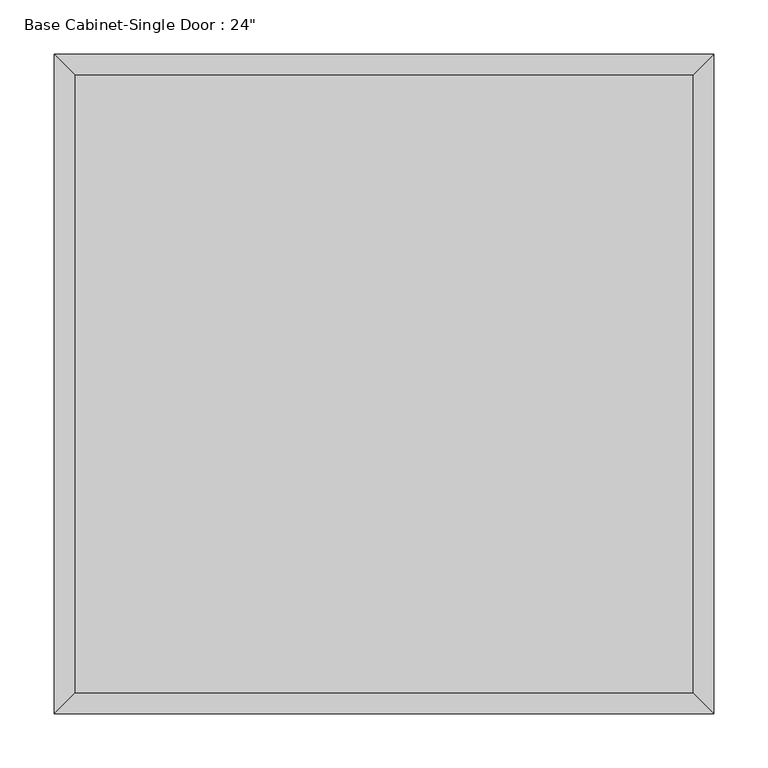
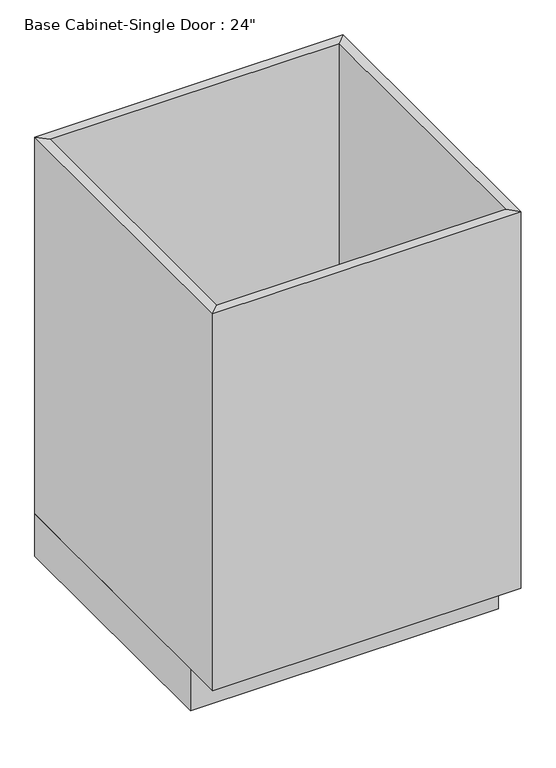
"""IFC4 building model written with IfcOpenShell, lengths in millimetres: furniture geometry."""

import ifcopenshell
import ifcopenshell.guid

model = None  # the IFC model being written
_history = None  # IfcOwnerHistory: only IFC2X3 demands one
_inside = {}  # id of a spatial element -> (the spatial element, [elements in it])
_under = {}  # id of a project, library or spatial element -> (it, [spatial elements below it])
_declared = {}  # id of a project -> (the project, [libraries it declares])
_typed = {}  # id of a type object -> (the type object, [elements of that type])
_made_of = {}  # id of a material, layer set ... -> (it, [elements and type objects made of it])


def new_model(schema):
    """Start an empty IFC model of exactly this schema.

    Asked for "IFC4X3", IfcOpenShell would pick the latest addendum, in which some entities
    have other attributes; the version numbers below select the first issue.
    IFC2X3 requires an IfcOwnerHistory on every rooted entity: one is made here for all.
    """
    global model, _history
    if schema == "IFC4X3":
        model = ifcopenshell.file(schema_version=(4, 3, 0, 0))
    else:
        model = ifcopenshell.file(schema=schema)
    _inside.clear()
    _under.clear()
    _declared.clear()
    _typed.clear()
    _made_of.clear()
    _history = None
    if model.schema == "IFC2X3":
        org = make("IfcOrganization", Name="unknown")
        user = make(
            "IfcPersonAndOrganization",
            ThePerson=make("IfcPerson", FamilyName="unknown"),
            TheOrganization=org,
        )
        app = make(
            "IfcApplication",
            ApplicationDeveloper=org,
            Version="unknown",
            ApplicationFullName="unknown",
            ApplicationIdentifier="unknown",
        )
        _history = make(
            "IfcOwnerHistory",
            OwningUser=user,
            OwningApplication=app,
            ChangeAction="ADDED",
            CreationDate=0,
        )
    return model


def make(cls, **values):
    """One entity of the class cls with the attributes given. An attribute that is None is left unset."""
    return model.create_entity(
        cls, **{name: value for name, value in values.items() if value is not None}
    )


def rooted(cls, **values):
    """An entity with a GlobalId (a new one), such as an element, a storey or a relation."""
    return make(cls, GlobalId=ifcopenshell.guid.new(), OwnerHistory=_history, **values)


def si_unit(unit_type, name, prefix=None):
    """IfcSIUnit, for example si_unit("LENGTHUNIT", "METRE", prefix="MILLI")."""
    return make("IfcSIUnit", UnitType=unit_type, Prefix=prefix, Name=name)


def assignment(units):
    """IfcUnitAssignment: the units of a project."""
    return None if units is None else make("IfcUnitAssignment", Units=units)


def point(xyz):
    """IfcCartesianPoint."""
    return None if xyz is None else make("IfcCartesianPoint", Coordinates=xyz)


def direction(xyz):
    """IfcDirection."""
    return None if xyz is None else make("IfcDirection", DirectionRatios=xyz)


def frame(location, z_axis=None, x_axis=None):
    """IfcAxis2Placement3D, a coordinate frame: its origin and axes. An axis left out is left unset."""
    return make(
        "IfcAxis2Placement3D",
        Location=point(location),
        Axis=direction(z_axis),
        RefDirection=direction(x_axis),
    )


def origin():
    """The frame at (0, 0, 0) with its axes left unset."""
    return frame((0.0, 0.0, 0.0))


def origin_with_axes():
    """The frame at (0, 0, 0) with the z axis (0, 0, 1) and the x axis (1, 0, 0) written out."""
    return frame((0.0, 0.0, 0.0), z_axis=(0.0, 0.0, 1.0), x_axis=(1.0, 0.0, 0.0))


def place(relative_to, where):
    """IfcLocalPlacement: puts the frame where relative to a parent placement (None: the world)."""
    return make(
        "IfcLocalPlacement", PlacementRelTo=relative_to, RelativePlacement=where
    )


def context(
    kind, dimensions, precision=None, world=None, true_north=None, identifier=None
):
    """IfcGeometricRepresentationContext, for example the 3D "Model" context."""
    return make(
        "IfcGeometricRepresentationContext",
        ContextIdentifier=identifier,
        ContextType=kind,
        CoordinateSpaceDimension=dimensions,
        Precision=precision,
        WorldCoordinateSystem=world,
        TrueNorth=true_north,
    )


def project(units=None, contexts=None):
    """IfcProject with its units and contexts."""
    return rooted(
        "IfcProject",
        Name="project",
        RepresentationContexts=contexts,
        UnitsInContext=assignment(units),
    )


def spatial(cls, under=None, at=None, **own):
    """A site, building, storey or space (cls), placed at a placement, below another one or the project."""
    s = rooted(cls, ObjectPlacement=at, **own)
    if under is not None:
        _under.setdefault(under.id(), (under, []))[1].append(s)
    return s


def polyline(points):
    """IfcPolyline through the points."""
    return make("IfcPolyline", Points=[point(p) for p in points])


def outline(outer, holes=None, kind="AREA"):
    """IfcArbitraryClosedProfileDef: a profile drawn as a closed curve; with holes, ...WithVoids."""
    if holes is None:
        return make("IfcArbitraryClosedProfileDef", ProfileType=kind, OuterCurve=outer)
    return make(
        "IfcArbitraryProfileDefWithVoids",
        ProfileType=kind,
        OuterCurve=outer,
        InnerCurves=holes,
    )


def extrude(swept, where, along, depth):
    """IfcExtrudedAreaSolid: the profile swept, set in the frame where, extruded along a direction by depth."""
    return make(
        "IfcExtrudedAreaSolid",
        SweptArea=swept,
        Position=where,
        ExtrudedDirection=direction(along),
        Depth=depth,
    )


def faces_of(points, faces, orient=None, outer=None):
    """IfcFace entities. A face is a list of loops; a loop is a list of indices into points, from 0.

    orient and outer hold one flag for each loop. By default every Orientation is true, the
    first loop of a face is its IfcFaceOuterBound and the others are IfcFaceBound.
    """
    made = []
    for i, loops in enumerate(faces):
        bounds = []
        for j, loop in enumerate(loops):
            is_outer = j == 0 if outer is None else outer[i][j]
            bounds.append(
                make(
                    "IfcFaceOuterBound" if is_outer else "IfcFaceBound",
                    Bound=make("IfcPolyLoop", Polygon=[points[k] for k in loop]),
                    Orientation=True if orient is None else orient[i][j],
                )
            )
        made.append(make("IfcFace", Bounds=bounds))
    return made


def faceted_brep(points, faces, orient=None, outer=None, voids=None):
    """IfcFacetedBrep: a solid bounded by flat faces; with voids (closed shells), ...WithVoids."""
    shared = [point(p) for p in points]
    hull = make("IfcClosedShell", CfsFaces=faces_of(shared, faces, orient, outer))
    if voids is None:
        return make("IfcFacetedBrep", Outer=hull)
    return make(
        "IfcFacetedBrepWithVoids",
        Outer=hull,
        Voids=[
            make(cls, CfsFaces=faces_of(shared, fs, o, b)) for cls, fs, o, b in voids
        ],
    )


def shape(context_of_items, identifier, shape_type, items):
    """IfcShapeRepresentation: the items that make up one representation, for example the "Body"."""
    return make(
        "IfcShapeRepresentation",
        ContextOfItems=context_of_items,
        RepresentationIdentifier=identifier,
        RepresentationType=shape_type,
        Items=items,
    )


def source(mapping_origin, context_of_items, identifier, shape_type, items):
    """IfcRepresentationMap: a shape defined once, which mapped items show again and again."""
    return make(
        "IfcRepresentationMap",
        MappingOrigin=mapping_origin,
        MappedRepresentation=shape(context_of_items, identifier, shape_type, items),
    )


def transform(
    local_origin,
    x_axis=None,
    y_axis=None,
    z_axis=None,
    scale=None,
    scale2=None,
    scale3=None,
    uniform=True,
):
    """IfcCartesianTransformationOperator3D, or its non-uniform kind. x_axis, y_axis, z_axis: its Axis1, 2, 3."""
    if uniform:
        return make(
            "IfcCartesianTransformationOperator3D",
            Axis1=direction(x_axis),
            Axis2=direction(y_axis),
            LocalOrigin=point(local_origin),
            Scale=scale,
            Axis3=direction(z_axis),
        )
    return make(
        "IfcCartesianTransformationOperator3DnonUniform",
        Axis1=direction(x_axis),
        Axis2=direction(y_axis),
        LocalOrigin=point(local_origin),
        Scale=scale,
        Axis3=direction(z_axis),
        Scale2=scale2,
        Scale3=scale3,
    )


def mapped(mapping_source, mapping_target):
    """IfcMappedItem: shows the shape of a source again, moved by a transform."""
    return make(
        "IfcMappedItem", MappingSource=mapping_source, MappingTarget=mapping_target
    )


def made_of(thing, what):
    """Note that an element or type object is made of a material, layer set ...; save() writes the relation."""
    if what is not None:
        _made_of.setdefault(what.id(), (what, []))[1].append(thing)
    return thing


def element(
    cls,
    number,
    at=None,
    inside=None,
    cuts=None,
    type_object=None,
    material=None,
    context=None,
    identifier="Body",
    shape_type=None,
    held_by="IfcProductDefinitionShape",
    body=None,
    shapes=None,
    **own,
):
    """One element of the class cls, such as IfcWall. Its Tag is "e" and its number.

    at: its placement. inside: the storey or other place that contains it. cuts: it is an
    opening in that element (IfcRelVoidsElement). A single representation is given by context,
    identifier, shape_type and body (its items); several are given by shapes. held_by: the class
    of the entity that holds the representations. save() writes the other relations.
    """
    e = rooted(cls, Tag="e%d" % number, ObjectPlacement=at, **own)
    if body is not None:
        shapes = [shape(context, identifier, shape_type, body)]
    if shapes is not None:
        e.Representation = make(held_by, Representations=shapes)
    if inside is not None:
        _inside.setdefault(inside.id(), (inside, []))[1].append(e)
    if cuts is not None:
        rooted(
            "IfcRelVoidsElement", RelatingBuildingElement=cuts, RelatedOpeningElement=e
        )
    if type_object is not None:
        _typed.setdefault(type_object.id(), (type_object, []))[1].append(e)
    return made_of(e, material)


def aggregate(whole, parts):
    """IfcRelAggregates: a whole, such as a stair, and the parts it consists of."""
    return rooted("IfcRelAggregates", RelatingObject=whole, RelatedObjects=parts)


def save(model, path):
    """Write the relations noted so far, then the file.

    IfcRelAggregates (storeys below a building ...), IfcRelContainedInSpatialStructure (elements
    in a storey), IfcRelDefinesByType, IfcRelAssociatesMaterial and IfcRelDeclares: one each for
    every whole, place, type object, material and project.
    """
    for whole, parts in _under.values():
        aggregate(whole, parts)
    for where, things in _inside.values():
        rooted(
            "IfcRelContainedInSpatialStructure",
            RelatedElements=things,
            RelatingStructure=where,
        )
    for kind, things in _typed.values():
        rooted("IfcRelDefinesByType", RelatedObjects=things, RelatingType=kind)
    for what, things in _made_of.values():
        rooted("IfcRelAssociatesMaterial", RelatedObjects=things, RelatingMaterial=what)
    for by, libraries in _declared.values():
        rooted("IfcRelDeclares", RelatingContext=by, RelatedDefinitions=libraries)
    model.write(path)


def furniture_222d96cf(model_context):
    return source(origin(), model_context, "Body", "SolidModel", [
        extrude(outline(polyline([(304.4877049, -19.05), (304.4877049, -590.55), (-267.0122951, -590.55), (-267.0122951, -19.05), (304.4877049, -19.05)])), frame((0.0, 0.0, 88.9), z_axis=(0.0, 0.0, 1.0), x_axis=(1.0, 0.0, 0.0)), (0.0, 0.0, 1.0), 19.05),
        faceted_brep([(304.4877049, -590.55, 876.3), (304.4877049, -590.55, 88.9), (-267.0122951, -590.55, 88.9), (-267.0122951, -590.55, 876.3), (323.5377049, -609.6, 876.3), (-286.0622951, -609.6, 876.3), (323.5377049, -609.6, 88.9), (-286.0622951, -609.6, 88.9), (-267.0122951, -19.05, 88.9), (-267.0122951, -19.05, 876.3), (-286.0622951, 0.0, 876.3), (-286.0622951, 0.0, 88.9), (304.4877049, -19.05, 88.9), (304.4877049, -19.05, 876.3), (323.5377049, 0.0, 876.3), (323.5377049, 0.0, 88.9)], [[[0, 1, 2, 3]], [[4, 0, 3, 5]], [[6, 4, 5, 7]], [[1, 6, 7, 2]], [[3, 2, 8, 9]], [[5, 3, 9, 10]], [[7, 5, 10, 11]], [[2, 7, 11, 8]], [[9, 8, 12, 13]], [[10, 9, 13, 14]], [[11, 10, 14, 15]], [[8, 11, 15, 12]], [[13, 12, 1, 0]], [[14, 13, 0, 4]], [[15, 14, 4, 6]], [[12, 15, 6, 1]]]),
        extrude(outline(polyline([(323.5377049, 0.0), (323.5377049, -533.4), (-286.0622951, -533.4), (-286.0622951, 0.0), (323.5377049, 0.0)])), origin_with_axes(), (0.0, 0.0, 1.0), 88.9),
    ])


if __name__ == "__main__":
    model = new_model("IFC4")
    model_context = context("Model", 3, world=origin())
    ifc_project = project(units=[si_unit("LENGTHUNIT", "METRE", prefix="MILLI")], contexts=[model_context])
    site = spatial("IfcSite", under=ifc_project)
    building = spatial("IfcBuilding", under=site)
    placement = place(None, origin())
    furniture_shape = furniture_222d96cf(model_context)
    element("IfcFurniture", 1, ObjectType="Base Cabinet-Single Door : 24\"", at=placement, inside=building, context=model_context, shape_type="MappedRepresentation", body=[
        mapped(furniture_shape, transform((0.0, 0.0, 0.0), x_axis=(1.0, 0.0, 0.0), y_axis=(0.0, 1.0, 0.0), z_axis=(0.0, 0.0, 1.0))),
    ])
    save(model, "model.ifc")

# Revit data of these elements
# Type "Base Cabinet-Single Door : 24\""
#   Depth = 2' - 0"
#   Height = 2' - 10 1/2"
#   Toe Depth = 0' - 3"
#   Toe Height = 0' - 3 1/2"
#   Width = 2' - 0"
# Element 1 (IfcFurniture, "Base Cabinet-Single Door : 24\"")
#   Materials on its faces: "Cabinet"
# Materials
#   "Cabinet": class "Wood", colour RGB 189 170 130, transparency 0, Cost = 0
